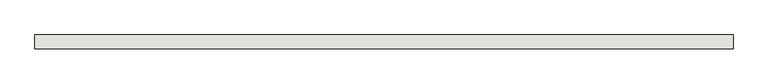
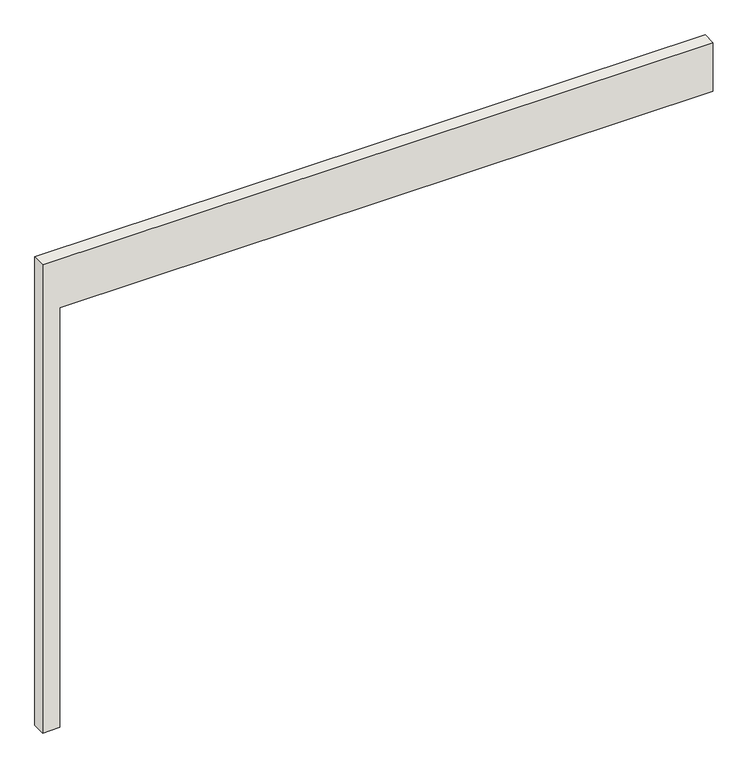
"""IFC4 building model written with IfcOpenShell, lengths in millimetres: wall geometry, 0_3d."""

from ifc_helpers import new_model, si_unit, frame, origin, place, context, project, spatial, polyline, outline, extrude, source, transform, mapped, element, save


def wall_0734cf4f(model_context):
    return source(origin(), model_context, "Body", "SweptSolid", [
        extrude(outline(polyline([(0.0, 100.0), (2580.0, 100.0), (2580.0, 3900.0), (2880.0, 3900.0), (2880.0, 0.0), (0.0, 0.0), (0.0, 100.0)])), frame((0.0, 0.0, 0.0), z_axis=(0.0, 1.0, 0.0), x_axis=(0.0, 0.0, 1.0)), (0.0, 0.0, 1.0), 78.0),
    ])


if __name__ == "__main__":
    model = new_model("IFC4")
    model_context = context("Model", 3, world=origin())
    ifc_project = project(units=[si_unit("LENGTHUNIT", "METRE", prefix="MILLI")], contexts=[model_context])
    site = spatial("IfcSite", under=ifc_project)
    building = spatial("IfcBuilding", under=site)
    placement = place(None, origin())
    wall_shape = wall_0734cf4f(model_context)
    element("IfcWall", 1, ObjectType="0_3d", at=placement, inside=building, context=model_context, shape_type="MappedRepresentation", body=[
        mapped(wall_shape, transform((0.0, 0.0, 0.0), x_axis=(1.0, 0.0, 0.0), y_axis=(0.0, 1.0, 0.0), z_axis=(0.0, 0.0, 1.0))),
    ])
    save(model, "model.ifc")

# Revit data of these elements
# Element 1 (IfcWall, "0_3d")
#   Materials on its faces: "glas"
# Materials
#   "glas": class "Unassigned", colour RGB 250 253 254, transparency 0.95
